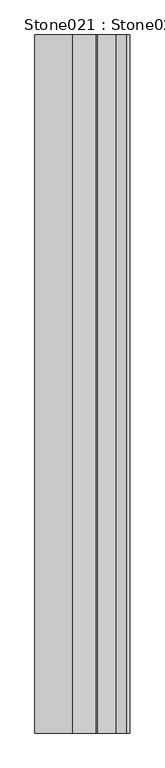
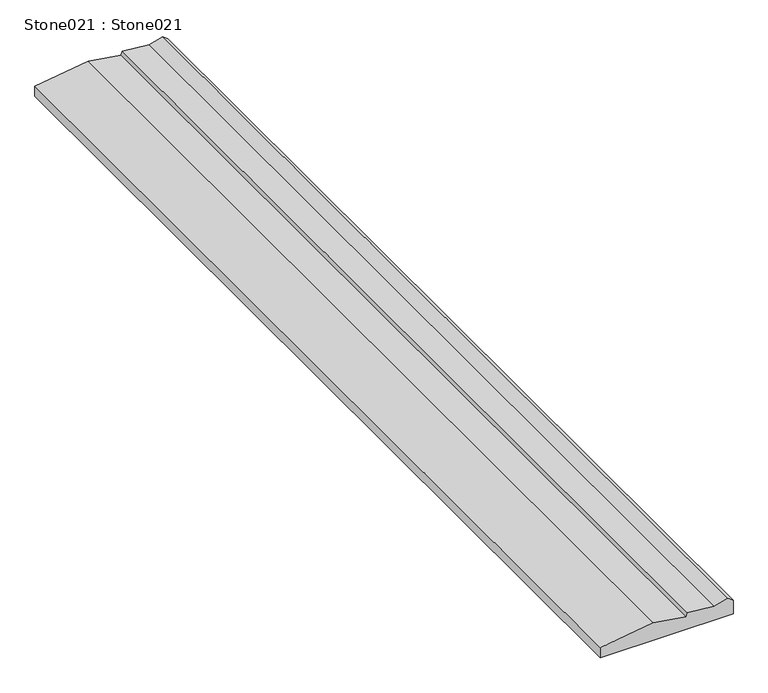
"""IFC4 building model written with IfcOpenShell, lengths in millimetres: proxy geometry, Stone021 : Stone021."""

from ifc_helpers import new_model, si_unit, frame, origin, place, context, project, spatial, polyline, outline, extrude, source, transform, mapped, element, save


def stone021_stone021_f7a2c303(model_context):
    return source(origin(), model_context, "Body", "SweptSolid", [
        extrude(outline(polyline([(33434.0234375, -10084.1142578), (33442.2773437, -10094.7001953), (33434.5546875, -10122.3896484), (33439.8789062, -10177.5029297), (33431.8945312, -10179.8994141), (33442.2773437, -10246.7275391), (33426.7905898, -10355.6966906), (33404.46875, -10355.6966906), (33404.46875, -10084.1142578), (33434.0234375, -10084.1142578)])), frame((0.0, 7182.1531721, 0.0), z_axis=(0.0, 1.0, 0.0), x_axis=(0.0, 0.0, 1.0)), (0.0, 0.0, 1.0), 2000.0),
    ])


if __name__ == "__main__":
    model = new_model("IFC4")
    model_context = context("Model", 3, world=origin())
    ifc_project = project(units=[si_unit("LENGTHUNIT", "METRE", prefix="MILLI")], contexts=[model_context])
    site = spatial("IfcSite", under=ifc_project)
    building = spatial("IfcBuilding", under=site)
    placement = place(None, origin())
    stone021_stone021_shape = stone021_stone021_f7a2c303(model_context)
    element("IfcBuildingElementProxy", 1, Name="Stone021 : Stone021", ObjectType="Stone021 : Stone021", at=placement, inside=building, context=model_context, shape_type="MappedRepresentation", body=[
        mapped(stone021_stone021_shape, transform((0.0, 0.0, 0.0), x_axis=(1.0, 0.0, 0.0), y_axis=(0.0, 1.0, 0.0), z_axis=(0.0, 0.0, 1.0))),
    ])
    save(model, "model.ifc")

# Revit data of these elements
# Type "Stone021 : Stone021"
#   NameOverride = "Stone021"
# Element 1 (IfcBuildingElementProxy, "Stone021 : Stone021")
#   Materials on its faces: "SPLIT FACE STONE"
# Materials
#   "SPLIT FACE STONE": class "Unassigned", colour RGB 205 195 181, transparency 0, Cost = 0
